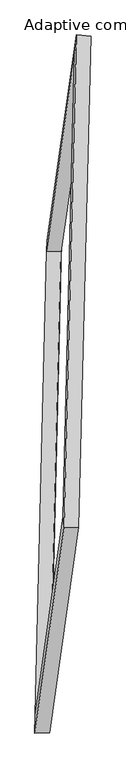
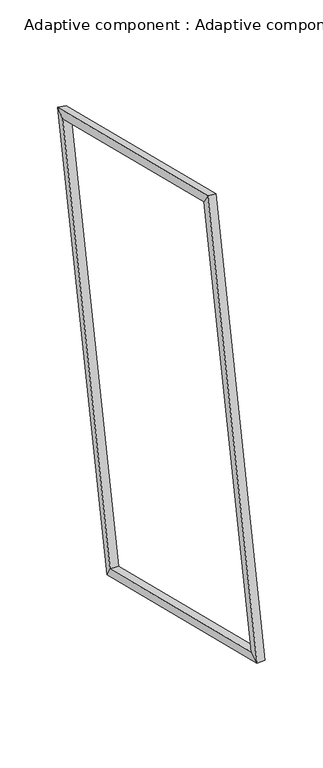
"""IFC4 building model written with IfcOpenShell, lengths in millimetres: proxy geometry, Adaptive component : Adaptive component."""

from ifc_helpers import new_model, si_unit, origin, place, context, project, spatial, faceted_brep, source, transform, mapped, element, save


def adaptive_component_adaptive_component_9a7f1c06(model_context):
    return source(origin(), model_context, "Body", "Brep", [
        faceted_brep([(65.3258355, 1052.6956044, 2693.0451197), (129.9919279, 1046.6971412, 2688.889198), (79.1157199, -1010.5060976, 3247.5423628), (14.2990527, -1010.5961946, 3253.3516911), (72.4559693, 1132.1749692, 2738.5669279), (18.3310939, -1056.3896537, 3332.8925297), (137.1220617, 1126.176506, 2734.4110061), (83.147761, -1056.2995567, 3327.0832014), (-46.8351781, -1889.3182961, -0.0955623), (-111.8879327, -1891.0556744, -0.373739), (-112.713419, -1970.7421381, -46.0840148), (-47.6606644, -1969.0047598, -45.8058382), (4.0410299, 167.8849428, -558.7487271), (-60.86115, 172.2361246, -560.6803103), (-58.5885436, 217.8224848, -640.4096166), (6.3136363, 213.471303, -638.4780334)], [[[0, 1, 2, 3]], [[4, 0, 3, 5]], [[6, 4, 5, 7]], [[1, 6, 7, 2]], [[3, 2, 8, 9]], [[5, 3, 9, 10]], [[7, 5, 10, 11]], [[2, 7, 11, 8]], [[9, 8, 12, 13]], [[10, 9, 13, 14]], [[11, 10, 14, 15]], [[8, 11, 15, 12]], [[13, 12, 1, 0]], [[14, 13, 0, 4]], [[15, 14, 4, 6]], [[12, 15, 6, 1]]]),
    ])


if __name__ == "__main__":
    model = new_model("IFC4")
    model_context = context("Model", 3, world=origin())
    ifc_project = project(units=[si_unit("LENGTHUNIT", "METRE", prefix="MILLI")], contexts=[model_context])
    site = spatial("IfcSite", under=ifc_project)
    building = spatial("IfcBuilding", under=site)
    placement = place(None, origin())
    adaptive_component_adaptive_component_shape = adaptive_component_adaptive_component_9a7f1c06(model_context)
    element("IfcBuildingElementProxy", 1, Name="Adaptive component : Adaptive component", ObjectType="Adaptive component : Adaptive component", at=placement, inside=building, context=model_context, shape_type="MappedRepresentation", body=[
        mapped(adaptive_component_adaptive_component_shape, transform((0.0, 0.0, 0.0), x_axis=(1.0, 0.0, 0.0), y_axis=(0.0, 1.0, 0.0), z_axis=(0.0, 0.0, 1.0))),
    ])
    save(model, "model.ifc")

# Revit data of these elements
# Type "Adaptive component : Adaptive component"
#   r [instance default] = 2063.125 mm
#   2r [instance default] = 4126.251 mm
#   Number [instance default] = 5
#   Default Elevation = 0
# Element 1 (IfcBuildingElementProxy, "Adaptive component : Adaptive component")
#   r = 2084.62 mm
#   2r = 4169.241 mm
